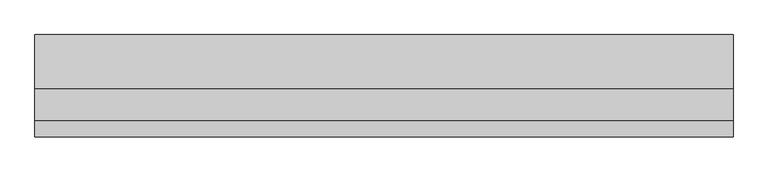
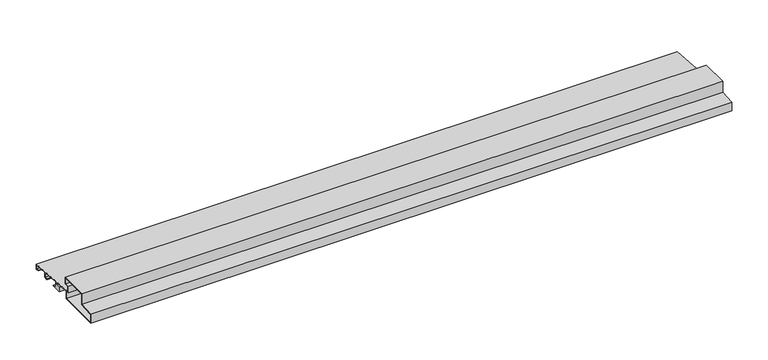
"""IFC4 building model written with IfcOpenShell, lengths in millimetres: proxy geometry, Generic Models 7:Generic Models 1:337419:Generic Models 1:337419 : Generic Models 7:Generic Models 1:337419:29 : Generic Models 7:Generic Models 1:337419:Generic Models 1:337419 : Generic Models 7:Generic Models 1:337419:301336."""

from ifc_helpers import new_model, si_unit, frame, origin, place, context, project, spatial, polyline, outline, extrude, source, transform, mapped, element, save


def generic_models_275a2bbb(model_context):
    return source(origin(), model_context, "Body", "SweptSolid", [
        extrude(outline(polyline([(-536611.070987, 17.7131392), (-536525.0520285, 11.6981076), (-536525.0520285, 3.1386095), (-536529.818116, 3.1386095), (-536529.818116, 4.5403999), (-536526.4661898, 4.5403999), (-536526.4661898, 10.391782), (-536547.7359627, 11.8791094), (-536547.7359627, 3.1386095), (-536553.9163918, 3.1386095), (-536553.9163918, 4.5403999), (-536549.1377531, 4.5403999), (-536549.1377531, 11.9771321), (-536577.8107393, 13.9821426), (-536577.8107393, 4.5403999), (-536571.3629263, 4.5403999), (-536571.3629263, 3.1353279), (-536587.4958368, 3.1353279), (-536587.4958368, 10.5307991), (-536579.2125297, 10.5307991), (-536579.2125297, 14.0801654), (-536606.8282273, 16.011243), (-536606.8282273, 3.1386095), (-536674.2770285, 3.1386095), (-536674.2770285, 17.7729935), (-536649.6257902, 19.496776), (-536649.6257902, 37.5825834), (-536604.1225858, 37.5825834), (-536604.1225858, 26.276657), (-536611.070987, 26.276657), (-536611.070987, 17.7131392)]), holes=[polyline([(-536608.4157273, 16.1222519), (-536612.658487, 16.4189345), (-536612.658487, 27.864157), (-536605.7100858, 27.864157), (-536605.7100858, 35.9950834), (-536648.0382902, 35.9950834), (-536648.0382902, 18.0164083), (-536672.6895285, 16.2926258), (-536672.6895285, 4.7261095), (-536608.4157273, 4.7261095), (-536608.4157273, 16.1222519)])]), frame((592715.7367242, 0.0, 0.0), z_axis=(1.0, 0.0, 0.0), x_axis=(0.0, 1.0, 0.0)), (0.0, 0.0, 1.0), 1016.0),
    ])


if __name__ == "__main__":
    model = new_model("IFC4")
    model_context = context("Model", 3, world=origin())
    ifc_project = project(units=[si_unit("LENGTHUNIT", "METRE", prefix="MILLI")], contexts=[model_context])
    site = spatial("IfcSite", under=ifc_project)
    building = spatial("IfcBuilding", under=site)
    placement = place(None, origin())
    generic_models_shape = generic_models_275a2bbb(model_context)
    element("IfcBuildingElementProxy", 1, Name="Generic Models 7:Generic Models 1:337419:Generic Models 1:337419 : Generic Models 7:Generic Models 1:337419:29 : Generic Models 7:Generic Models 1:337419:Generic Models 1:337419 : Generic Models 7:Generic Models 1:337419:301336", ObjectType="Generic Models 7:Generic Models 1:337419:Generic Models 1:337419 : Generic Models 7:Generic Models 1:337419:29 : Generic Models 7:Generic Models 1:337419:Generic Models 1:337419 : Generic Models 7:Generic Models 1:337419:301336", at=placement, inside=building, context=model_context, shape_type="MappedRepresentation", body=[
        mapped(generic_models_shape, transform((0.0, 0.0, 0.0), x_axis=(1.0, 0.0, 0.0), y_axis=(0.0, 1.0, 0.0), z_axis=(0.0, 0.0, 1.0))),
    ])
    save(model, "model.ifc")

# Revit data of these elements
# Type "Generic Models 7:Generic Models 1:337419:Generic Models 1:337419 : Generic Models 7:Generic Models 1:337419:29 : Generic Models 7:Generic Models 1:337419:Generic Models 1:337419 : Generic Models 7:Generic Models 1:337419:301336"
#   NameOverride = "Generic Models 7:Generic Models 1:337419:Generic Models 1:337419 : Generic Models 7:Generic Models 1:337419:301336"
#   ObjectTypeOverride = "Generic Models 1:337419 : Generic Models 7:Generic Models 1:337419"
#   Reference = "Generic Models 1"
#   Tag = "301336"
# Element 1 (IfcBuildingElementProxy, "Generic Models 7:Generic Models 1:337419:Generic Models 1:337419 : Generic Models 7:Generic Models 1:337419:29 : Generic Models 7:Generic Models 1:337419:Generic Models 1:337419 : Generic Models 7:Generic Models 1:337419:301336")
#   Materials on its faces: "DOOR THRESHOLD - SEE DOOR SCHEDULE"
# Materials
#   "DOOR THRESHOLD - SEE DOOR SCHEDULE": class "Generic", colour RGB 233 233 233, transparency 0, Cost = 0
